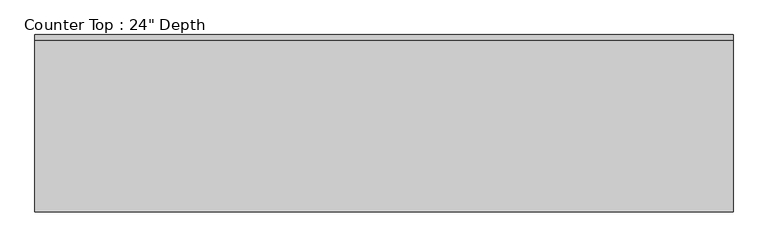
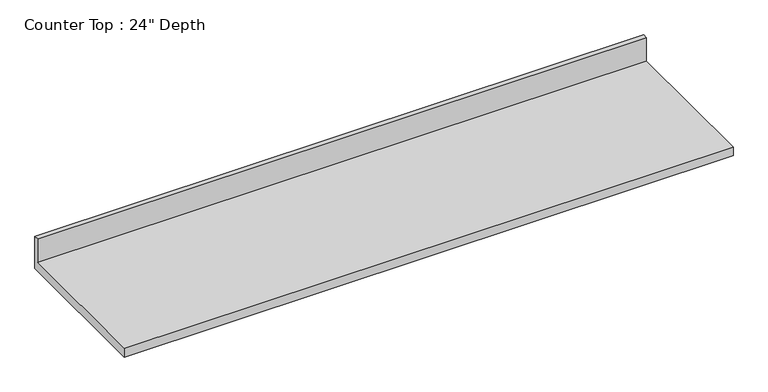
"""IFC4 building model written with IfcOpenShell, lengths in millimetres: furniture geometry."""

from ifc_helpers import new_model, si_unit, frame, origin, place, context, project, spatial, polyline, outline, extrude, source, transform, mapped, element, save


def furniture_01140236(model_context):
    return source(origin(), model_context, "Body", "SweptSolid", [
        extrude(outline(polyline([(0.0, 1016.0), (0.0, 876.3), (-635.0, 876.3), (-635.0, 914.4), (-19.05, 914.4), (-19.05, 1016.0), (0.0, 1016.0)])), frame((-1200.4622951, 0.0, 0.0), z_axis=(1.0, 0.0, 0.0), x_axis=(0.0, 1.0, 0.0)), (0.0, 0.0, 1.0), 2497.1375),
    ])


if __name__ == "__main__":
    model = new_model("IFC4")
    model_context = context("Model", 3, world=origin())
    ifc_project = project(units=[si_unit("LENGTHUNIT", "METRE", prefix="MILLI")], contexts=[model_context])
    site = spatial("IfcSite", under=ifc_project)
    building = spatial("IfcBuilding", under=site)
    placement = place(None, origin())
    furniture_shape = furniture_01140236(model_context)
    element("IfcFurniture", 1, ObjectType="Counter Top : 24\" Depth", at=placement, inside=building, context=model_context, shape_type="MappedRepresentation", body=[
        mapped(furniture_shape, transform((0.0, 0.0, 0.0), x_axis=(1.0, 0.0, 0.0), y_axis=(0.0, 1.0, 0.0), z_axis=(0.0, 0.0, 1.0))),
    ])
    save(model, "model.ifc")

# Revit data of these elements
# Project information
#   Project Issue Date = "Issue Date"
#   Project Status = "Project Status"
#   Client Name = "Owner"
#   Project Address = "Enter address here"
#   Project Name = "Project Name"
#   Project Number = "Project Number"
# Type "Counter Top : 24\" Depth"
#   Assembly Code = "C1030400"
#   Counter Thickness = 0' - 1 1/2"
#   Depth = 2' - 1"
#   Height = 3' - 0"
#   Length [instance default] = 8' - 0"
#   Counter Top Material = none
# Element 1 (IfcFurniture, "Counter Top : 24\" Depth")
#   Length = 8' - 2 5/16"
#   Materials on its faces: "Counter Top"
# Materials
#   "Counter Top": class "Wood", colour RGB 226 177 128, transparency 0, Cost = 0
